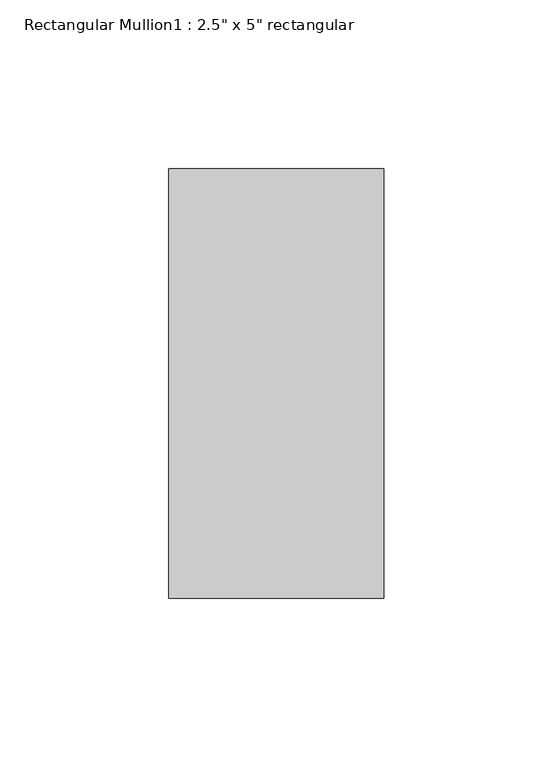
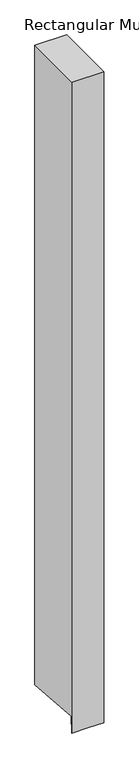
"""IFC4 building model written with IfcOpenShell, lengths in millimetres: member geometry."""

from ifc_helpers import new_model, si_unit, origin, place, context, project, spatial, faceted_brep, source, transform, mapped, element, save


def member_275a0903(model_context):
    return source(origin(), model_context, "Body", "Brep", [
        faceted_brep([(31.75, 63.5, 0.0), (-31.75, 63.5, 0.0), (-31.75, -63.5, 0.0), (31.75, -63.5, 0.0), (31.75, 63.5, -1344.0500431), (0.0, 63.5, -1344.0500431), (-31.75, 63.5, -1344.0500431), (-31.75, -60.9736199, -1334.8041085), (-31.75, -63.5, -1368.815562), (0.0, -63.5, -1368.815562), (31.75, -63.5, -1368.815562), (31.75, -60.9736199, -1334.8041085), (0.0, -60.9736199, -1334.8041085)], [[[0, 1, 2, 3]], [[1, 0, 4, 5, 6]], [[2, 1, 6, 7, 8]], [[3, 2, 8, 9, 10]], [[0, 3, 10, 11, 4]], [[4, 11, 12, 5]], [[11, 10, 9, 12]], [[9, 8, 7, 12]], [[7, 6, 5, 12]]]),
    ])


if __name__ == "__main__":
    model = new_model("IFC4")
    model_context = context("Model", 3, world=origin())
    ifc_project = project(units=[si_unit("LENGTHUNIT", "METRE", prefix="MILLI")], contexts=[model_context])
    site = spatial("IfcSite", under=ifc_project)
    building = spatial("IfcBuilding", under=site)
    placement = place(None, origin())
    member_shape = member_275a0903(model_context)
    element("IfcMember", 1, ObjectType="Rectangular Mullion1 : 2.5\" x 5\" rectangular", at=placement, inside=building, context=model_context, shape_type="MappedRepresentation", body=[
        mapped(member_shape, transform((0.0, 0.0, 0.0), x_axis=(1.0, 0.0, 0.0), y_axis=(0.0, 1.0, 0.0), z_axis=(0.0, 0.0, 1.0))),
    ])
    save(model, "model.ifc")

# Revit data of these elements
# Type "Rectangular Mullion1 : 2.5\" x 5\" rectangular"
#   built-in parameter 1007304 = 0.416667 (stored number, unit not read)
#   built-in parameter 1007301 = 0.104167 (stored number, unit not read)
#   built-in parameter 1007300 = 0.104167 (stored number, unit not read)
# Element 1 (IfcMember, "Rectangular Mullion1 : 2.5\" x 5\" rectangular")
#   Materials on its faces: "support-frame"
# Materials
#   "support-frame": class "Unassigned", colour RGB 233 233 233, transparency 0, Cost = 0
